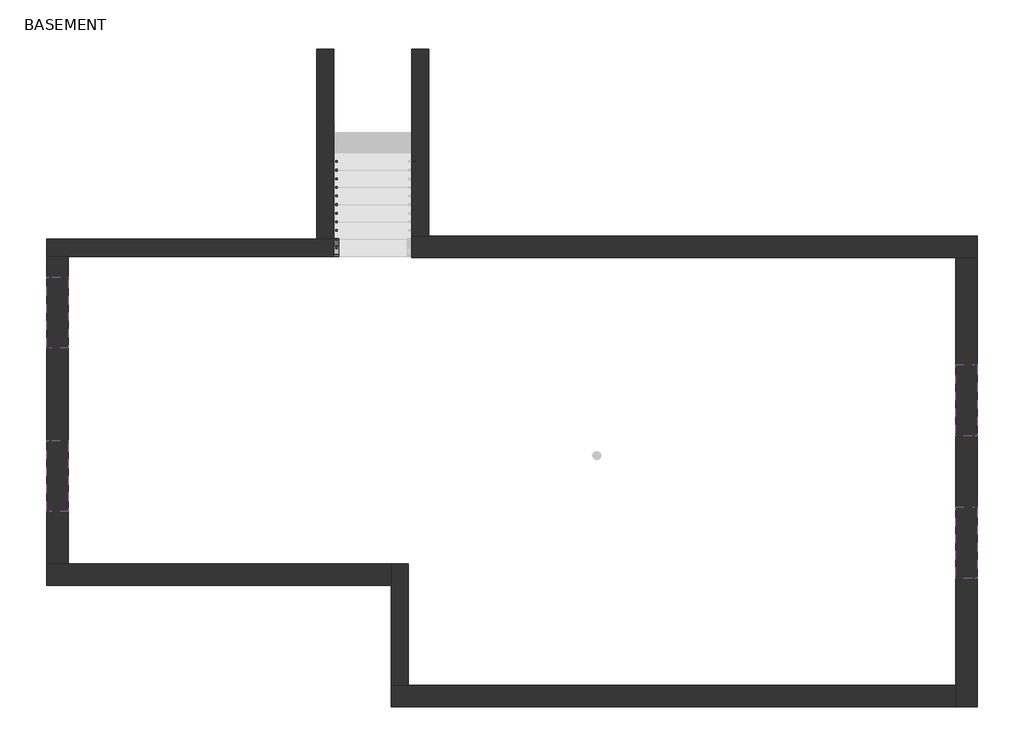
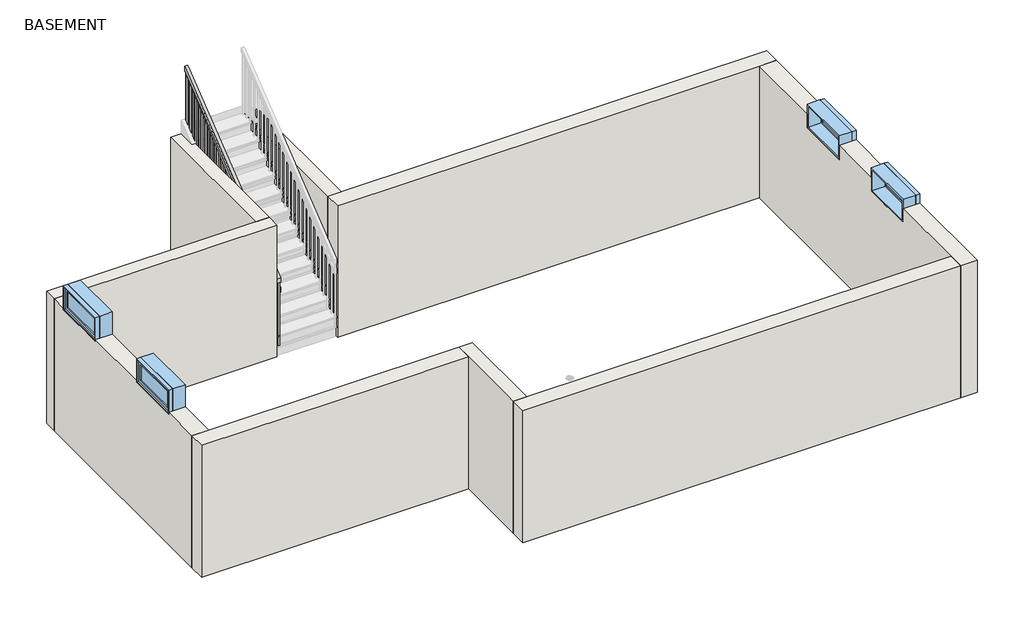
# One storey, part 1 of 2: 9 walls, 4 windows, 2 railings.
"""IFC4 building model written with IfcOpenShell, lengths in millimetres."""

import ifcopenshell
import ifcopenshell.guid

model = None  # the IFC model being written
_history = None  # IfcOwnerHistory: only IFC2X3 demands one
_inside = {}  # id of a spatial element -> (the spatial element, [elements in it])
_under = {}  # id of a project, library or spatial element -> (it, [spatial elements below it])
_declared = {}  # id of a project -> (the project, [libraries it declares])
_typed = {}  # id of a type object -> (the type object, [elements of that type])
_made_of = {}  # id of a material, layer set ... -> (it, [elements and type objects made of it])


def new_model(schema):
    """Start an empty IFC model of exactly this schema.

    Asked for "IFC4X3", IfcOpenShell would pick the latest addendum, in which some entities
    have other attributes; the version numbers below select the first issue.
    IFC2X3 requires an IfcOwnerHistory on every rooted entity: one is made here for all.
    """
    global model, _history
    if schema == "IFC4X3":
        model = ifcopenshell.file(schema_version=(4, 3, 0, 0))
    else:
        model = ifcopenshell.file(schema=schema)
    _inside.clear()
    _under.clear()
    _declared.clear()
    _typed.clear()
    _made_of.clear()
    _history = None
    if model.schema == "IFC2X3":
        org = make("IfcOrganization", Name="unknown")
        user = make(
            "IfcPersonAndOrganization",
            ThePerson=make("IfcPerson", FamilyName="unknown"),
            TheOrganization=org,
        )
        app = make(
            "IfcApplication",
            ApplicationDeveloper=org,
            Version="unknown",
            ApplicationFullName="unknown",
            ApplicationIdentifier="unknown",
        )
        _history = make(
            "IfcOwnerHistory",
            OwningUser=user,
            OwningApplication=app,
            ChangeAction="ADDED",
            CreationDate=0,
        )
    return model


def make(cls, **values):
    """One entity of the class cls with the attributes given. An attribute that is None is left unset."""
    return model.create_entity(
        cls, **{name: value for name, value in values.items() if value is not None}
    )


def rooted(cls, **values):
    """An entity with a GlobalId (a new one), such as an element, a storey or a relation."""
    return make(cls, GlobalId=ifcopenshell.guid.new(), OwnerHistory=_history, **values)


def si_unit(unit_type, name, prefix=None):
    """IfcSIUnit, for example si_unit("LENGTHUNIT", "METRE", prefix="MILLI")."""
    return make("IfcSIUnit", UnitType=unit_type, Prefix=prefix, Name=name)


def assignment(units):
    """IfcUnitAssignment: the units of a project."""
    return None if units is None else make("IfcUnitAssignment", Units=units)


def point(xyz):
    """IfcCartesianPoint."""
    return None if xyz is None else make("IfcCartesianPoint", Coordinates=xyz)


def direction(xyz):
    """IfcDirection."""
    return None if xyz is None else make("IfcDirection", DirectionRatios=xyz)


def frame(location, z_axis=None, x_axis=None):
    """IfcAxis2Placement3D, a coordinate frame: its origin and axes. An axis left out is left unset."""
    return make(
        "IfcAxis2Placement3D",
        Location=point(location),
        Axis=direction(z_axis),
        RefDirection=direction(x_axis),
    )


def origin():
    """The frame at (0, 0, 0) with its axes left unset."""
    return frame((0.0, 0.0, 0.0))


def place(relative_to, where):
    """IfcLocalPlacement: puts the frame where relative to a parent placement (None: the world)."""
    return make(
        "IfcLocalPlacement", PlacementRelTo=relative_to, RelativePlacement=where
    )


def context(
    kind, dimensions, precision=None, world=None, true_north=None, identifier=None
):
    """IfcGeometricRepresentationContext, for example the 3D "Model" context."""
    return make(
        "IfcGeometricRepresentationContext",
        ContextIdentifier=identifier,
        ContextType=kind,
        CoordinateSpaceDimension=dimensions,
        Precision=precision,
        WorldCoordinateSystem=world,
        TrueNorth=true_north,
    )


def project(units=None, contexts=None):
    """IfcProject with its units and contexts."""
    return rooted(
        "IfcProject",
        Name="project",
        RepresentationContexts=contexts,
        UnitsInContext=assignment(units),
    )


def spatial(cls, under=None, at=None, **own):
    """A site, building, storey or space (cls), placed at a placement, below another one or the project."""
    s = rooted(cls, ObjectPlacement=at, **own)
    if under is not None:
        _under.setdefault(under.id(), (under, []))[1].append(s)
    return s


def polyline(points):
    """IfcPolyline through the points."""
    return make("IfcPolyline", Points=[point(p) for p in points])


def outline(outer, holes=None, kind="AREA"):
    """IfcArbitraryClosedProfileDef: a profile drawn as a closed curve; with holes, ...WithVoids."""
    if holes is None:
        return make("IfcArbitraryClosedProfileDef", ProfileType=kind, OuterCurve=outer)
    return make(
        "IfcArbitraryProfileDefWithVoids",
        ProfileType=kind,
        OuterCurve=outer,
        InnerCurves=holes,
    )


def extrude(swept, where, along, depth):
    """IfcExtrudedAreaSolid: the profile swept, set in the frame where, extruded along a direction by depth."""
    return make(
        "IfcExtrudedAreaSolid",
        SweptArea=swept,
        Position=where,
        ExtrudedDirection=direction(along),
        Depth=depth,
    )


def faces_of(points, faces, orient=None, outer=None):
    """IfcFace entities. A face is a list of loops; a loop is a list of indices into points, from 0.

    orient and outer hold one flag for each loop. By default every Orientation is true, the
    first loop of a face is its IfcFaceOuterBound and the others are IfcFaceBound.
    """
    made = []
    for i, loops in enumerate(faces):
        bounds = []
        for j, loop in enumerate(loops):
            is_outer = j == 0 if outer is None else outer[i][j]
            bounds.append(
                make(
                    "IfcFaceOuterBound" if is_outer else "IfcFaceBound",
                    Bound=make("IfcPolyLoop", Polygon=[points[k] for k in loop]),
                    Orientation=True if orient is None else orient[i][j],
                )
            )
        made.append(make("IfcFace", Bounds=bounds))
    return made


def faceted_brep(points, faces, orient=None, outer=None, voids=None):
    """IfcFacetedBrep: a solid bounded by flat faces; with voids (closed shells), ...WithVoids."""
    shared = [point(p) for p in points]
    hull = make("IfcClosedShell", CfsFaces=faces_of(shared, faces, orient, outer))
    if voids is None:
        return make("IfcFacetedBrep", Outer=hull)
    return make(
        "IfcFacetedBrepWithVoids",
        Outer=hull,
        Voids=[
            make(cls, CfsFaces=faces_of(shared, fs, o, b)) for cls, fs, o, b in voids
        ],
    )


def shape(context_of_items, identifier, shape_type, items):
    """IfcShapeRepresentation: the items that make up one representation, for example the "Body"."""
    return make(
        "IfcShapeRepresentation",
        ContextOfItems=context_of_items,
        RepresentationIdentifier=identifier,
        RepresentationType=shape_type,
        Items=items,
    )


def source(mapping_origin, context_of_items, identifier, shape_type, items):
    """IfcRepresentationMap: a shape defined once, which mapped items show again and again."""
    return make(
        "IfcRepresentationMap",
        MappingOrigin=mapping_origin,
        MappedRepresentation=shape(context_of_items, identifier, shape_type, items),
    )


def transform(
    local_origin,
    x_axis=None,
    y_axis=None,
    z_axis=None,
    scale=None,
    scale2=None,
    scale3=None,
    uniform=True,
):
    """IfcCartesianTransformationOperator3D, or its non-uniform kind. x_axis, y_axis, z_axis: its Axis1, 2, 3."""
    if uniform:
        return make(
            "IfcCartesianTransformationOperator3D",
            Axis1=direction(x_axis),
            Axis2=direction(y_axis),
            LocalOrigin=point(local_origin),
            Scale=scale,
            Axis3=direction(z_axis),
        )
    return make(
        "IfcCartesianTransformationOperator3DnonUniform",
        Axis1=direction(x_axis),
        Axis2=direction(y_axis),
        LocalOrigin=point(local_origin),
        Scale=scale,
        Axis3=direction(z_axis),
        Scale2=scale2,
        Scale3=scale3,
    )


def mapped(mapping_source, mapping_target):
    """IfcMappedItem: shows the shape of a source again, moved by a transform."""
    return make(
        "IfcMappedItem", MappingSource=mapping_source, MappingTarget=mapping_target
    )


def made_of(thing, what):
    """Note that an element or type object is made of a material, layer set ...; save() writes the relation."""
    if what is not None:
        _made_of.setdefault(what.id(), (what, []))[1].append(thing)
    return thing


def element(
    cls,
    number,
    at=None,
    inside=None,
    cuts=None,
    type_object=None,
    material=None,
    context=None,
    identifier="Body",
    shape_type=None,
    held_by="IfcProductDefinitionShape",
    body=None,
    shapes=None,
    **own,
):
    """One element of the class cls, such as IfcWall. Its Tag is "e" and its number.

    at: its placement. inside: the storey or other place that contains it. cuts: it is an
    opening in that element (IfcRelVoidsElement). A single representation is given by context,
    identifier, shape_type and body (its items); several are given by shapes. held_by: the class
    of the entity that holds the representations. save() writes the other relations.
    """
    e = rooted(cls, Tag="e%d" % number, ObjectPlacement=at, **own)
    if body is not None:
        shapes = [shape(context, identifier, shape_type, body)]
    if shapes is not None:
        e.Representation = make(held_by, Representations=shapes)
    if inside is not None:
        _inside.setdefault(inside.id(), (inside, []))[1].append(e)
    if cuts is not None:
        rooted(
            "IfcRelVoidsElement", RelatingBuildingElement=cuts, RelatedOpeningElement=e
        )
    if type_object is not None:
        _typed.setdefault(type_object.id(), (type_object, []))[1].append(e)
    return made_of(e, material)


def aggregate(whole, parts):
    """IfcRelAggregates: a whole, such as a stair, and the parts it consists of."""
    return rooted("IfcRelAggregates", RelatingObject=whole, RelatedObjects=parts)


def save(model, path):
    """Write the relations noted so far, then the file.

    IfcRelAggregates (storeys below a building ...), IfcRelContainedInSpatialStructure (elements
    in a storey), IfcRelDefinesByType, IfcRelAssociatesMaterial and IfcRelDeclares: one each for
    every whole, place, type object, material and project.
    """
    for whole, parts in _under.values():
        aggregate(whole, parts)
    for where, things in _inside.values():
        rooted(
            "IfcRelContainedInSpatialStructure",
            RelatedElements=things,
            RelatingStructure=where,
        )
    for kind, things in _typed.values():
        rooted("IfcRelDefinesByType", RelatedObjects=things, RelatingType=kind)
    for what, things in _made_of.values():
        rooted("IfcRelAssociatesMaterial", RelatedObjects=things, RelatingMaterial=what)
    for by, libraries in _declared.values():
        rooted("IfcRelDeclares", RelatingContext=by, RelatedDefinitions=libraries)
    model.write(path)


def window_bf5cd34b(model_context):
    return source(origin(), model_context, "Body", "SweptSolid", [
        extrude(outline(polyline([(317.5, 79.375), (-393.7, 79.375), (-393.7, 92.075), (317.5, 92.075), (317.5, 79.375)])), frame((0.0, 0.0, 977.9), z_axis=(0.0, 0.0, 1.0), x_axis=(1.0, 0.0, 0.0)), (0.0, 0.0, 1.0), 254.0),
        extrude(outline(polyline([(1276.35, -438.15), (933.45, -438.15), (933.45, 361.95), (1276.35, 361.95), (1276.35, -438.15)]), holes=[polyline([(1231.9, -393.7), (1231.9, 317.5), (977.9, 317.5), (977.9, -393.7), (1231.9, -393.7)])]), frame((0.0, 63.5, 0.0), z_axis=(0.0, 1.0, 0.0), x_axis=(0.0, 0.0, 1.0)), (0.0, 0.0, 1.0), 44.45),
        extrude(outline(polyline([(1295.4, -457.2), (914.4, -457.2), (914.4, 381.0), (1295.4, 381.0), (1295.4, -457.2)]), holes=[polyline([(1263.65, -425.45), (1263.65, 349.25), (946.15, 349.25), (946.15, -425.45), (1263.65, -425.45)])]), frame((0.0, -127.0, 0.0), z_axis=(0.0, 1.0, 0.0), x_axis=(0.0, 0.0, 1.0)), (0.0, 0.0, 1.0), 190.5),
        extrude(outline(polyline([(1295.4, 381.0), (1295.4, -457.2), (914.4, -457.2), (914.4, 381.0), (1295.4, 381.0)]), holes=[polyline([(1276.35, 361.95), (933.45, 361.95), (933.45, -438.15), (1276.35, -438.15), (1276.35, 361.95)])]), frame((0.0, 63.5, 0.0), z_axis=(0.0, 1.0, 0.0), x_axis=(0.0, 0.0, 1.0)), (0.0, 0.0, 1.0), 63.5),
    ])


model = new_model("IFC4")

# Units and contexts
model_context = context("Model", 3, world=origin())
ifc_project = project(units=[si_unit("LENGTHUNIT", "METRE", prefix="MILLI")], contexts=[model_context])

# Site, building, storey
site = spatial("IfcSite", under=ifc_project)
building = spatial("IfcBuilding", under=site)
storey = spatial("IfcBuildingStorey", under=building, Name="BASEMENT", Elevation=-2266.95)

# Railings
placement = place(None, origin())
element("IfcRailing", 1, ObjectType="Handrail - Rectangular", at=placement, inside=storey, context=model_context, shape_type="SweptSolid", body=[
    extrude(outline(polyline([(-12572.2570712, -1084.7503866), (-12572.2570712, -1019.9076923), (-10133.8570712, 914.4), (-10133.8570712, 849.5573057), (-12572.2570712, -1084.7503866)])), frame((-25042.4664763, 0.0, 0.0), z_axis=(1.0, 0.0, 0.0), x_axis=(0.0, 1.0, 0.0)), (0.0, 0.0, 1.0), 50.8),
    extrude(outline(polyline([(-10225.9320712, 776.5170413), (-10225.9320712, -161.1923077), (-10244.9820712, -161.1923077), (-10244.9820712, 761.4052624), (-10225.9320712, 776.5170413)])), frame((-25026.5914763, 0.0, 0.0), z_axis=(1.0, 0.0, 0.0), x_axis=(0.0, 1.0, 0.0)), (0.0, 0.0, 1.0), 19.05),
    extrude(outline(polyline([(-10327.5320712, 695.9208874), (-10327.5320712, -161.1923077), (-10346.5820712, -161.1923077), (-10346.5820712, 680.8091086), (-10327.5320712, 695.9208874)])), frame((-25026.5914763, 0.0, 0.0), z_axis=(1.0, 0.0, 0.0), x_axis=(0.0, 1.0, 0.0)), (0.0, 0.0, 1.0), 19.05),
    extrude(outline(polyline([(-10429.1320712, 615.3247336), (-10429.1320712, -322.3846154), (-10448.1820712, -322.3846154), (-10448.1820712, 600.2129547), (-10429.1320712, 615.3247336)])), frame((-25026.5914763, 0.0, 0.0), z_axis=(1.0, 0.0, 0.0), x_axis=(0.0, 1.0, 0.0)), (0.0, 0.0, 1.0), 19.05),
    extrude(outline(polyline([(-10530.7320712, 534.7285797), (-10530.7320712, -322.3846154), (-10549.7820712, -322.3846154), (-10549.7820712, 519.6168009), (-10530.7320712, 534.7285797)])), frame((-25026.5914763, 0.0, 0.0), z_axis=(1.0, 0.0, 0.0), x_axis=(0.0, 1.0, 0.0)), (0.0, 0.0, 1.0), 19.05),
    extrude(outline(polyline([(-10632.3320712, 454.1324259), (-10632.3320712, -483.5769231), (-10651.3820712, -483.5769231), (-10651.3820712, 439.020647), (-10632.3320712, 454.1324259)])), frame((-25026.5914763, 0.0, 0.0), z_axis=(1.0, 0.0, 0.0), x_axis=(0.0, 1.0, 0.0)), (0.0, 0.0, 1.0), 19.05),
    extrude(outline(polyline([(-10733.9320712, 373.536272), (-10733.9320712, -483.5769231), (-10752.9820712, -483.5769231), (-10752.9820712, 358.4244932), (-10733.9320712, 373.536272)])), frame((-25026.5914763, 0.0, 0.0), z_axis=(1.0, 0.0, 0.0), x_axis=(0.0, 1.0, 0.0)), (0.0, 0.0, 1.0), 19.05),
    extrude(outline(polyline([(-10835.5320712, 292.9401182), (-10835.5320712, -644.7692308), (-10854.5820712, -644.7692308), (-10854.5820712, 277.8283394), (-10835.5320712, 292.9401182)])), frame((-25026.5914763, 0.0, 0.0), z_axis=(1.0, 0.0, 0.0), x_axis=(0.0, 1.0, 0.0)), (0.0, 0.0, 1.0), 19.05),
    extrude(outline(polyline([(-10937.1320712, 212.3439644), (-10937.1320712, -644.7692308), (-10956.1820712, -644.7692308), (-10956.1820712, 197.2321855), (-10937.1320712, 212.3439644)])), frame((-25026.5914763, 0.0, 0.0), z_axis=(1.0, 0.0, 0.0), x_axis=(0.0, 1.0, 0.0)), (0.0, 0.0, 1.0), 19.05),
    extrude(outline(polyline([(-11038.7320712, 131.7478105), (-11038.7320712, -805.9615385), (-11057.7820712, -805.9615385), (-11057.7820712, 116.6360317), (-11038.7320712, 131.7478105)])), frame((-25026.5914763, 0.0, 0.0), z_axis=(1.0, 0.0, 0.0), x_axis=(0.0, 1.0, 0.0)), (0.0, 0.0, 1.0), 19.05),
    extrude(outline(polyline([(-11140.3320712, 51.1516567), (-11140.3320712, -805.9615385), (-11159.3820712, -805.9615385), (-11159.3820712, 36.0398778), (-11140.3320712, 51.1516567)])), frame((-25026.5914763, 0.0, 0.0), z_axis=(1.0, 0.0, 0.0), x_axis=(0.0, 1.0, 0.0)), (0.0, 0.0, 1.0), 19.05),
    extrude(outline(polyline([(-11241.9320712, -29.4444972), (-11241.9320712, -967.1538462), (-11260.9820712, -967.1538462), (-11260.9820712, -44.556276), (-11241.9320712, -29.4444972)])), frame((-25026.5914763, 0.0, 0.0), z_axis=(1.0, 0.0, 0.0), x_axis=(0.0, 1.0, 0.0)), (0.0, 0.0, 1.0), 19.05),
    extrude(outline(polyline([(-11343.5320712, -110.040651), (-11343.5320712, -967.1538462), (-11362.5820712, -967.1538462), (-11362.5820712, -125.1524299), (-11343.5320712, -110.040651)])), frame((-25026.5914763, 0.0, 0.0), z_axis=(1.0, 0.0, 0.0), x_axis=(0.0, 1.0, 0.0)), (0.0, 0.0, 1.0), 19.05),
    extrude(outline(polyline([(-11445.1320712, -190.6368049), (-11445.1320712, -1128.3461538), (-11464.1820712, -1128.3461538), (-11464.1820712, -205.7485837), (-11445.1320712, -190.6368049)])), frame((-25026.5914763, 0.0, 0.0), z_axis=(1.0, 0.0, 0.0), x_axis=(0.0, 1.0, 0.0)), (0.0, 0.0, 1.0), 19.05),
    extrude(outline(polyline([(-11546.7320712, -271.2329587), (-11546.7320712, -1128.3461538), (-11565.7820712, -1128.3461538), (-11565.7820712, -286.3447376), (-11546.7320712, -271.2329587)])), frame((-25026.5914763, 0.0, 0.0), z_axis=(1.0, 0.0, 0.0), x_axis=(0.0, 1.0, 0.0)), (0.0, 0.0, 1.0), 19.05),
    extrude(outline(polyline([(-11648.3320712, -351.8291126), (-11648.3320712, -1289.5384615), (-11667.3820712, -1289.5384615), (-11667.3820712, -366.9408914), (-11648.3320712, -351.8291126)])), frame((-25026.5914763, 0.0, 0.0), z_axis=(1.0, 0.0, 0.0), x_axis=(0.0, 1.0, 0.0)), (0.0, 0.0, 1.0), 19.05),
    extrude(outline(polyline([(-11749.9320712, -432.4252664), (-11749.9320712, -1289.5384615), (-11768.9820712, -1289.5384615), (-11768.9820712, -447.5370453), (-11749.9320712, -432.4252664)])), frame((-25026.5914763, 0.0, 0.0), z_axis=(1.0, 0.0, 0.0), x_axis=(0.0, 1.0, 0.0)), (0.0, 0.0, 1.0), 19.05),
    extrude(outline(polyline([(-11851.5320712, -513.0214203), (-11851.5320712, -1450.7307692), (-11870.5820712, -1450.7307692), (-11870.5820712, -528.1331991), (-11851.5320712, -513.0214203)])), frame((-25026.5914763, 0.0, 0.0), z_axis=(1.0, 0.0, 0.0), x_axis=(0.0, 1.0, 0.0)), (0.0, 0.0, 1.0), 19.05),
    extrude(outline(polyline([(-11953.1320712, -593.6175741), (-11953.1320712, -1450.7307692), (-11972.1820712, -1450.7307692), (-11972.1820712, -608.729353), (-11953.1320712, -593.6175741)])), frame((-25026.5914763, 0.0, 0.0), z_axis=(1.0, 0.0, 0.0), x_axis=(0.0, 1.0, 0.0)), (0.0, 0.0, 1.0), 19.05),
    extrude(outline(polyline([(-12054.7320712, -674.213728), (-12054.7320712, -1611.9230769), (-12073.7820712, -1611.9230769), (-12073.7820712, -689.3255068), (-12054.7320712, -674.213728)])), frame((-25026.5914763, 0.0, 0.0), z_axis=(1.0, 0.0, 0.0), x_axis=(0.0, 1.0, 0.0)), (0.0, 0.0, 1.0), 19.05),
    extrude(outline(polyline([(-12156.3320712, -754.8098818), (-12156.3320712, -1611.9230769), (-12175.3820712, -1611.9230769), (-12175.3820712, -769.9216606), (-12156.3320712, -754.8098818)])), frame((-25026.5914763, 0.0, 0.0), z_axis=(1.0, 0.0, 0.0), x_axis=(0.0, 1.0, 0.0)), (0.0, 0.0, 1.0), 19.05),
    extrude(outline(polyline([(-12257.9320712, -835.4060356), (-12257.9320712, -1773.1153846), (-12276.9820712, -1773.1153846), (-12276.9820712, -850.5178145), (-12257.9320712, -835.4060356)])), frame((-25026.5914763, 0.0, 0.0), z_axis=(1.0, 0.0, 0.0), x_axis=(0.0, 1.0, 0.0)), (0.0, 0.0, 1.0), 19.05),
    extrude(outline(polyline([(-12359.5320712, -916.0021895), (-12359.5320712, -1773.1153846), (-12378.5820712, -1773.1153846), (-12378.5820712, -931.1139683), (-12359.5320712, -916.0021895)])), frame((-25026.5914763, 0.0, 0.0), z_axis=(1.0, 0.0, 0.0), x_axis=(0.0, 1.0, 0.0)), (0.0, 0.0, 1.0), 19.05),
    extrude(outline(polyline([(-12461.1320712, -996.5983433), (-12461.1320712, -1934.3076923), (-12480.1820712, -1934.3076923), (-12480.1820712, -1011.7101222), (-12461.1320712, -996.5983433)])), frame((-25026.5914763, 0.0, 0.0), z_axis=(1.0, 0.0, 0.0), x_axis=(0.0, 1.0, 0.0)), (0.0, 0.0, 1.0), 19.05),
    extrude(outline(polyline([(-10133.8570712, 849.5573057), (-10133.8570712, -161.1923077), (-10152.9070712, -161.1923077), (-10152.9070712, 834.4455269), (-10133.8570712, 849.5573057)])), frame((-25026.5914763, 0.0, 0.0), z_axis=(1.0, 0.0, 0.0), x_axis=(0.0, 1.0, 0.0)), (0.0, 0.0, 1.0), 19.05),
    extrude(outline(polyline([(-12553.2070712, -1069.6386078), (-12553.2070712, -1934.3076923), (-12572.2570712, -1934.3076923), (-12572.2570712, -1084.7503866), (-12553.2070712, -1069.6386078)])), frame((-25026.5914763, 0.0, 0.0), z_axis=(1.0, 0.0, 0.0), x_axis=(0.0, 1.0, 0.0)), (0.0, 0.0, 1.0), 19.05),
])
element("IfcRailing", 2, ObjectType="Handrail - Rectangular", at=placement, inside=storey, context=model_context, shape_type="SweptSolid", body=[
    extrude(outline(polyline([(-12572.2570712, -1245.110853), (-12572.2570712, -1178.1692308), (-10133.8570712, 914.4), (-10133.8570712, 847.4583777), (-12572.2570712, -1245.110853)])), frame((-25042.4664763, 0.0, 0.0), z_axis=(1.0, 0.0, 0.0), x_axis=(0.0, 1.0, 0.0)), (0.0, 0.0, 1.0), 50.8),
    extrude(outline(polyline([(-10225.9320712, 768.4420917), (-10225.9320712, -174.3807692), (-10244.9820712, -174.3807692), (-10244.9820712, 752.0938946), (-10225.9320712, 768.4420917)])), frame((-25026.5914763, 0.0, 0.0), z_axis=(1.0, 0.0, 0.0), x_axis=(0.0, 1.0, 0.0)), (0.0, 0.0, 1.0), 19.05),
    extrude(outline(polyline([(-10327.5320712, 681.2517071), (-10327.5320712, -174.3807692), (-10346.5820712, -174.3807692), (-10346.5820712, 664.9035099), (-10327.5320712, 681.2517071)])), frame((-25026.5914763, 0.0, 0.0), z_axis=(1.0, 0.0, 0.0), x_axis=(0.0, 1.0, 0.0)), (0.0, 0.0, 1.0), 19.05),
    extrude(outline(polyline([(-10429.1320712, 594.0613224), (-10429.1320712, -348.7615385), (-10448.1820712, -348.7615385), (-10448.1820712, 577.7131253), (-10429.1320712, 594.0613224)])), frame((-25026.5914763, 0.0, 0.0), z_axis=(1.0, 0.0, 0.0), x_axis=(0.0, 1.0, 0.0)), (0.0, 0.0, 1.0), 19.05),
    extrude(outline(polyline([(-10530.7320712, 506.8709378), (-10530.7320712, -348.7615385), (-10549.7820712, -348.7615385), (-10549.7820712, 490.5227407), (-10530.7320712, 506.8709378)])), frame((-25026.5914763, 0.0, 0.0), z_axis=(1.0, 0.0, 0.0), x_axis=(0.0, 1.0, 0.0)), (0.0, 0.0, 1.0), 19.05),
    extrude(outline(polyline([(-10632.3320712, 419.6805532), (-10632.3320712, -523.1423077), (-10651.3820712, -523.1423077), (-10651.3820712, 403.3323561), (-10632.3320712, 419.6805532)])), frame((-25026.5914763, 0.0, 0.0), z_axis=(1.0, 0.0, 0.0), x_axis=(0.0, 1.0, 0.0)), (0.0, 0.0, 1.0), 19.05),
    extrude(outline(polyline([(-10733.9320712, 332.4901686), (-10733.9320712, -523.1423077), (-10752.9820712, -523.1423077), (-10752.9820712, 316.1419715), (-10733.9320712, 332.4901686)])), frame((-25026.5914763, 0.0, 0.0), z_axis=(1.0, 0.0, 0.0), x_axis=(0.0, 1.0, 0.0)), (0.0, 0.0, 1.0), 19.05),
    extrude(outline(polyline([(-10835.5320712, 245.299784), (-10835.5320712, -697.5230769), (-10854.5820712, -697.5230769), (-10854.5820712, 228.9515869), (-10835.5320712, 245.299784)])), frame((-25026.5914763, 0.0, 0.0), z_axis=(1.0, 0.0, 0.0), x_axis=(0.0, 1.0, 0.0)), (0.0, 0.0, 1.0), 19.05),
    extrude(outline(polyline([(-10937.1320712, 158.1093994), (-10937.1320712, -697.5230769), (-10956.1820712, -697.5230769), (-10956.1820712, 141.7612022), (-10937.1320712, 158.1093994)])), frame((-25026.5914763, 0.0, 0.0), z_axis=(1.0, 0.0, 0.0), x_axis=(0.0, 1.0, 0.0)), (0.0, 0.0, 1.0), 19.05),
    extrude(outline(polyline([(-11038.7320712, 70.9190147), (-11038.7320712, -871.9038462), (-11057.7820712, -871.9038462), (-11057.7820712, 54.5708176), (-11038.7320712, 70.9190147)])), frame((-25026.5914763, 0.0, 0.0), z_axis=(1.0, 0.0, 0.0), x_axis=(0.0, 1.0, 0.0)), (0.0, 0.0, 1.0), 19.05),
    extrude(outline(polyline([(-11140.3320712, -16.2713699), (-11140.3320712, -871.9038462), (-11159.3820712, -871.9038462), (-11159.3820712, -32.619567), (-11140.3320712, -16.2713699)])), frame((-25026.5914763, 0.0, 0.0), z_axis=(1.0, 0.0, 0.0), x_axis=(0.0, 1.0, 0.0)), (0.0, 0.0, 1.0), 19.05),
    extrude(outline(polyline([(-11241.9320712, -103.4617545), (-11241.9320712, -1046.2846154), (-11260.9820712, -1046.2846154), (-11260.9820712, -119.8099516), (-11241.9320712, -103.4617545)])), frame((-25026.5914763, 0.0, 0.0), z_axis=(1.0, 0.0, 0.0), x_axis=(0.0, 1.0, 0.0)), (0.0, 0.0, 1.0), 19.05),
    extrude(outline(polyline([(-11343.5320712, -190.6521391), (-11343.5320712, -1046.2846154), (-11362.5820712, -1046.2846154), (-11362.5820712, -207.0003362), (-11343.5320712, -190.6521391)])), frame((-25026.5914763, 0.0, 0.0), z_axis=(1.0, 0.0, 0.0), x_axis=(0.0, 1.0, 0.0)), (0.0, 0.0, 1.0), 19.05),
    extrude(outline(polyline([(-11445.1320712, -277.8425237), (-11445.1320712, -1220.6653846), (-11464.1820712, -1220.6653846), (-11464.1820712, -294.1907208), (-11445.1320712, -277.8425237)])), frame((-25026.5914763, 0.0, 0.0), z_axis=(1.0, 0.0, 0.0), x_axis=(0.0, 1.0, 0.0)), (0.0, 0.0, 1.0), 19.05),
    extrude(outline(polyline([(-11546.7320712, -365.0329083), (-11546.7320712, -1220.6653846), (-11565.7820712, -1220.6653846), (-11565.7820712, -381.3811054), (-11546.7320712, -365.0329083)])), frame((-25026.5914763, 0.0, 0.0), z_axis=(1.0, 0.0, 0.0), x_axis=(0.0, 1.0, 0.0)), (0.0, 0.0, 1.0), 19.05),
    extrude(outline(polyline([(-11648.3320712, -452.2232929), (-11648.3320712, -1395.0461538), (-11667.3820712, -1395.0461538), (-11667.3820712, -468.5714901), (-11648.3320712, -452.2232929)])), frame((-25026.5914763, 0.0, 0.0), z_axis=(1.0, 0.0, 0.0), x_axis=(0.0, 1.0, 0.0)), (0.0, 0.0, 1.0), 19.05),
    extrude(outline(polyline([(-11749.9320712, -539.4136776), (-11749.9320712, -1395.0461538), (-11768.9820712, -1395.0461538), (-11768.9820712, -555.7618747), (-11749.9320712, -539.4136776)])), frame((-25026.5914763, 0.0, 0.0), z_axis=(1.0, 0.0, 0.0), x_axis=(0.0, 1.0, 0.0)), (0.0, 0.0, 1.0), 19.05),
    extrude(outline(polyline([(-11851.5320712, -626.6040622), (-11851.5320712, -1569.4269231), (-11870.5820712, -1569.4269231), (-11870.5820712, -642.9522593), (-11851.5320712, -626.6040622)])), frame((-25026.5914763, 0.0, 0.0), z_axis=(1.0, 0.0, 0.0), x_axis=(0.0, 1.0, 0.0)), (0.0, 0.0, 1.0), 19.05),
    extrude(outline(polyline([(-11953.1320712, -713.7944468), (-11953.1320712, -1569.4269231), (-11972.1820712, -1569.4269231), (-11972.1820712, -730.1426439), (-11953.1320712, -713.7944468)])), frame((-25026.5914763, 0.0, 0.0), z_axis=(1.0, 0.0, 0.0), x_axis=(0.0, 1.0, 0.0)), (0.0, 0.0, 1.0), 19.05),
    extrude(outline(polyline([(-12054.7320712, -800.9848314), (-12054.7320712, -1743.8076923), (-12073.7820712, -1743.8076923), (-12073.7820712, -817.3330285), (-12054.7320712, -800.9848314)])), frame((-25026.5914763, 0.0, 0.0), z_axis=(1.0, 0.0, 0.0), x_axis=(0.0, 1.0, 0.0)), (0.0, 0.0, 1.0), 19.05),
    extrude(outline(polyline([(-12156.3320712, -888.175216), (-12156.3320712, -1743.8076923), (-12175.3820712, -1743.8076923), (-12175.3820712, -904.5234131), (-12156.3320712, -888.175216)])), frame((-25026.5914763, 0.0, 0.0), z_axis=(1.0, 0.0, 0.0), x_axis=(0.0, 1.0, 0.0)), (0.0, 0.0, 1.0), 19.05),
    extrude(outline(polyline([(-12257.9320712, -975.3656006), (-12257.9320712, -1918.1884615), (-12276.9820712, -1918.1884615), (-12276.9820712, -991.7137978), (-12257.9320712, -975.3656006)])), frame((-25026.5914763, 0.0, 0.0), z_axis=(1.0, 0.0, 0.0), x_axis=(0.0, 1.0, 0.0)), (0.0, 0.0, 1.0), 19.05),
    extrude(outline(polyline([(-12359.5320712, -1062.5559853), (-12359.5320712, -1918.1884615), (-12378.5820712, -1918.1884615), (-12378.5820712, -1078.9041824), (-12359.5320712, -1062.5559853)])), frame((-25026.5914763, 0.0, 0.0), z_axis=(1.0, 0.0, 0.0), x_axis=(0.0, 1.0, 0.0)), (0.0, 0.0, 1.0), 19.05),
    extrude(outline(polyline([(-12461.1320712, -1149.7463699), (-12461.1320712, -2092.5692308), (-12480.1820712, -2092.5692308), (-12480.1820712, -1166.094567), (-12461.1320712, -1149.7463699)])), frame((-25026.5914763, 0.0, 0.0), z_axis=(1.0, 0.0, 0.0), x_axis=(0.0, 1.0, 0.0)), (0.0, 0.0, 1.0), 19.05),
    extrude(outline(polyline([(-10133.8570712, 847.4583777), (-10133.8570712, -174.3807692), (-10152.9070712, -174.3807692), (-10152.9070712, 831.1101806), (-10133.8570712, 847.4583777)])), frame((-25026.5914763, 0.0, 0.0), z_axis=(1.0, 0.0, 0.0), x_axis=(0.0, 1.0, 0.0)), (0.0, 0.0, 1.0), 19.05),
    extrude(outline(polyline([(-12553.2070712, -1228.7626559), (-12553.2070712, -2092.5692308), (-12572.2570712, -2092.5692308), (-12572.2570712, -1245.110853), (-12553.2070712, -1228.7626559)])), frame((-25026.5914763, 0.0, 0.0), z_axis=(1.0, 0.0, 0.0), x_axis=(0.0, 1.0, 0.0)), (0.0, 0.0, 1.0), 19.05),
])

# Walls
element("IfcWall", 3, ObjectType="Generic - 10\"", at=placement, inside=storey, context=model_context, shape_type="Brep", body=[
    faceted_brep([(-17733.6164763, -12584.9570712, -2266.95), (-17733.6164763, -17620.5070712, -2266.95), (-17733.6164763, -17874.5070712, -2266.95), (-17733.6164763, -17874.5070712, -152.4), (-17733.6164763, -17620.5070712, -152.4), (-17733.6164763, -16361.0904046, -152.4), (-17733.6164763, -16361.0904046, -381.0), (-17733.6164763, -15522.8904046, -381.0), (-17733.6164763, -15522.8904046, -152.4), (-17733.6164763, -14682.5737379, -152.4), (-17733.6164763, -14682.5737379, -381.0), (-17733.6164763, -13844.3737379, -381.0), (-17733.6164763, -13844.3737379, -152.4), (-17733.6164763, -12584.9570712, -152.4), (-17479.6164763, -17874.5070712, -2266.95), (-17479.6164763, -12584.9570712, -2266.95), (-17479.6164763, -12584.9570712, -152.4), (-17479.6164763, -13844.3737379, -152.4), (-17479.6164763, -13844.3737379, -381.0), (-17479.6164763, -14682.5737379, -381.0), (-17479.6164763, -14682.5737379, -152.4), (-17479.6164763, -15522.8904046, -152.4), (-17479.6164763, -15522.8904046, -381.0), (-17479.6164763, -16361.0904046, -381.0), (-17479.6164763, -16361.0904046, -152.4), (-17479.6164763, -17874.5070712, -152.4)], [[[0, 1, 2, 3, 4, 5, 6, 7, 8, 9, 10, 11, 12, 13]], [[14, 15, 16, 17, 18, 19, 20, 21, 22, 23, 24, 25]], [[2, 1, 0, 15, 14]], [[0, 13, 16, 15]], [[3, 2, 14, 25]], [[3, 25, 24, 5, 4]], [[8, 21, 20, 9]], [[16, 13, 12, 17]], [[23, 6, 5, 24]], [[6, 23, 22, 7]], [[7, 22, 21, 8]], [[19, 10, 9, 20]], [[10, 19, 18, 11]], [[11, 18, 17, 12]]]),
])
element("IfcWall", 4, ObjectType="Generic - 10\"", at=placement, inside=storey, context=model_context, shape_type="Brep", body=[
    faceted_brep([(-17733.6164763, -17620.5070712, -2266.95), (-24172.5164763, -17620.5070712, -2266.95), (-24375.7164763, -17620.5070712, -2266.95), (-24375.7164763, -17620.5070712, -152.4), (-24172.5164763, -17620.5070712, -152.4), (-17733.6164763, -17620.5070712, -152.4), (-17733.6164763, -17874.5070712, -2266.95), (-17733.6164763, -17874.5070712, -152.4), (-24375.7164763, -17874.5070712, -152.4), (-24375.7164763, -17874.5070712, -2266.95)], [[[0, 1, 2, 3, 4, 5]], [[6, 7, 8, 9]], [[2, 1, 0, 6, 9]], [[0, 5, 7, 6]], [[3, 2, 9, 8]], [[5, 4, 3, 8, 7]]]),
])
element("IfcWall", 5, ObjectType="Generic - 10\"", at=placement, inside=storey, context=model_context, shape_type="Brep", body=[
    faceted_brep([(-24375.7164763, -16191.7570712, -2266.95), (-28173.0164763, -16191.7570712, -2266.95), (-28427.0164763, -16191.7570712, -2266.95), (-28427.0164763, -16191.7570712, -152.4), (-28173.0164763, -16191.7570712, -152.4), (-24375.7164763, -16191.7570712, -152.4), (-24375.7164763, -16445.7570712, -2266.95), (-24375.7164763, -16445.7570712, -152.4), (-25734.6164763, -16445.7570712, -152.4), (-28427.0164763, -16445.7570712, -152.4), (-28427.0164763, -16445.7570712, -2266.95)], [[[0, 1, 2, 3, 4, 5]], [[6, 7, 8, 9, 10]], [[2, 1, 0, 6, 10]], [[0, 5, 7, 6]], [[3, 2, 10, 9]], [[5, 4, 3, 9, 8, 7]]]),
])
element("IfcWall", 6, ObjectType="Generic - 10\"", at=placement, inside=storey, context=model_context, shape_type="SweptSolid", body=[
    extrude(outline(polyline([(-12572.2570712, -2266.95), (-16191.7570712, -2266.95), (-16191.7570712, -152.4), (-15575.8070712, -152.4), (-15575.8070712, -177.7746), (-14737.6070712, -177.7746), (-14737.6070712, -152.4), (-13651.7570712, -152.4), (-13651.7570712, -177.7746), (-12813.5570712, -177.7746), (-12813.5570712, -152.4), (-12572.2570712, -152.4), (-12572.2570712, -2266.95)])), frame((-28427.0164763, 0.0, 0.0), z_axis=(1.0, 0.0, 0.0), x_axis=(0.0, 1.0, 0.0)), (0.0, 0.0, 1.0), 254.0),
])
element("IfcWall", 7, ObjectType="Generic - 10\"", at=placement, inside=storey, context=model_context, shape_type="Brep", body=[
    faceted_brep([(-24134.4164763, -12584.9570712, -2266.95), (-17733.6164763, -12584.9570712, -2266.95), (-17479.6164763, -12584.9570712, -2266.95), (-17479.6164763, -12584.9570712, -152.4), (-17733.6164763, -12584.9570712, -152.4), (-24134.4164763, -12584.9570712, -152.4), (-24134.4164763, -12330.9570712, -2266.95), (-24134.4164763, -12330.9570712, -152.4), (-23931.2164763, -12330.9570712, -152.4), (-17479.6164763, -12330.9570712, -152.4), (-17479.6164763, -12330.9570712, -2266.95), (-23931.2164763, -12330.9570712, -2266.95)], [[[0, 1, 2, 3, 4, 5]], [[6, 7, 8, 9, 10, 11]], [[2, 1, 0, 6, 11, 10]], [[3, 2, 10, 9]], [[0, 5, 7, 6]], [[5, 4, 3, 9, 8, 7]]]),
])
element("IfcWall", 8, ObjectType="Generic - 8\"", at=placement, inside=storey, context=model_context, shape_type="Brep", body=[
    faceted_brep([(-28427.0164763, -12572.2570712, -2266.95), (-28173.0164763, -12572.2570712, -2266.95), (-25048.8164763, -12572.2570712, -2266.95), (-25048.8164763, -12572.2570712, -152.4), (-28173.0164763, -12572.2570712, -152.4), (-28427.0164763, -12572.2570712, -152.4), (-28427.0164763, -12369.0570712, -2266.95), (-28427.0164763, -12369.0570712, -152.4), (-25252.0164763, -12369.0570712, -152.4), (-25048.8164763, -12369.0570712, -152.4), (-25048.8164763, -12369.0570712, -2266.95), (-25252.0164763, -12369.0570712, -2266.95)], [[[0, 1, 2, 3, 4, 5]], [[6, 7, 8, 9, 10, 11]], [[2, 1, 0, 6, 11, 10]], [[0, 5, 7, 6]], [[3, 2, 10, 9]], [[5, 4, 3, 9, 8, 7]]]),
])
element("IfcWall", 9, ObjectType="Generic - 8\"", at=placement, inside=storey, context=model_context, shape_type="Brep", body=[
    faceted_brep([(-24172.5164763, -17620.5070712, -2266.95), (-24172.5164763, -16191.7570712, -2266.95), (-24172.5164763, -16191.7570712, -152.4), (-24172.5164763, -17620.5070712, -152.4), (-24375.7164763, -17620.5070712, -2266.95), (-24375.7164763, -17620.5070712, -152.4), (-24375.7164763, -16445.7570712, -152.4), (-24375.7164763, -16191.7570712, -152.4), (-24375.7164763, -16191.7570712, -2266.95), (-24375.7164763, -16445.7570712, -2266.95)], [[[0, 1, 2, 3]], [[4, 5, 6, 7, 8, 9]], [[1, 0, 4, 9, 8]], [[0, 3, 5, 4]], [[2, 1, 8, 7]], [[3, 2, 7, 6, 5]]]),
])
element("IfcWall", 10, ObjectType="Generic - 8\"", at=placement, inside=storey, context=model_context, shape_type="SweptSolid", body=[
    extrude(outline(polyline([(-25048.8164763, -10133.8570712), (-25048.8164763, -12369.0570712), (-25252.0164763, -12369.0570712), (-25252.0164763, -10133.8570712), (-25048.8164763, -10133.8570712)])), frame((0.0, 0.0, -2266.95), z_axis=(0.0, 0.0, 1.0), x_axis=(1.0, 0.0, 0.0)), (0.0, 0.0, 1.0), 2114.55),
])
element("IfcWall", 11, ObjectType="Generic - 8\"", at=placement, inside=storey, context=model_context, shape_type="SweptSolid", body=[
    extrude(outline(polyline([(-24134.4164763, -12330.9570712), (-24134.4164763, -10133.8570712), (-23931.2164763, -10133.8570712), (-23931.2164763, -12330.9570712), (-24134.4164763, -12330.9570712)])), frame((0.0, 0.0, -2266.95), z_axis=(0.0, 0.0, 1.0), x_axis=(1.0, 0.0, 0.0)), (0.0, 0.0, 1.0), 2114.55),
])

# Windows
window_shape = window_bf5cd34b(model_context)
element("IfcWindow", 12, ObjectType="Fixed1 : 2'-9\" x 1'-3\"", at=placement, inside=storey, context=model_context, shape_type="MappedRepresentation", body=[
    mapped(window_shape, transform((-28300.0164763, -15118.6070712, -1092.1746), x_axis=(0.0, 1.0, 0.0), y_axis=(-1.0, 0.0, 0.0), z_axis=(0.0, 0.0, 1.0))),
])
element("IfcWindow", 13, ObjectType="Fixed1 : 2'-9\" x 1'-3\"", at=placement, inside=storey, context=model_context, shape_type="MappedRepresentation", body=[
    mapped(window_shape, transform((-28300.0164763, -13194.5570712, -1092.1746), x_axis=(0.0, 1.0, 0.0), y_axis=(-1.0, 0.0, 0.0), z_axis=(0.0, 0.0, 1.0))),
])
element("IfcWindow", 14, ObjectType="Fixed1 : 2'-9\" x 1'-3\"", at=placement, inside=storey, context=model_context, shape_type="MappedRepresentation", body=[
    mapped(window_shape, transform((-17606.6164763, -14301.5737379, -1295.4), x_axis=(0.0, -1.0, 0.0), y_axis=(1.0, 0.0, 0.0), z_axis=(0.0, 0.0, 1.0))),
])
element("IfcWindow", 15, ObjectType="Fixed1 : 2'-9\" x 1'-3\"", at=placement, inside=storey, context=model_context, shape_type="MappedRepresentation", body=[
    mapped(window_shape, transform((-17606.6164763, -15980.0904046, -1295.4), x_axis=(0.0, -1.0, 0.0), y_axis=(1.0, 0.0, 0.0), z_axis=(0.0, 0.0, 1.0))),
])

save(model, "model.ifc")

# Revit data of these elements
# Project information
#   Project Issue Date = "06/12/2018"
#   Project Status = "Project Status"
#   Client Name = "Owner"
#   Project Address = "5253 KING JAMES WAY, FITCHBURG, WI"
#   Project Name = "FORAGE KOMBUCHA"
#   Project Number = "Project Number"
# Grids (mm)
#   "B": line (-20559.366, -20036.147) -> (-20559.366, -11545.141)
#   "C": line (-23277.166, -20036.147) -> (-23277.166, -11545.141)
#   "D": line (-25994.966, -20036.147) -> (-25994.966, -11545.141)
# Type "Handrail - Rectangular"
#   Assembly Code = "C2010400"
#   built-in parameter 1008612 = 0.0416667 (stored number, unit not read)
#   built-in parameter 1008611 = 0.0416667 (stored number, unit not read)
#   built-in parameter 1008609 = 0.333333 (stored number, unit not read)
#   built-in parameter 1008604 = 0.166667 (stored number, unit not read)
#   built-in parameter 1008603 = 0.166667 (stored number, unit not read)
#   Railing Height = 3' - 0"
#   built-in parameter 1008630 = 2
#   built-in parameter 1008610 = 2
#   built-in parameter 1008618 = Baluster - Square : 3/4"
# Type "Generic - 10\""
#   Assembly Code = "B2010"
#   Layers, outside or top first: 0' - 10" no material (function 1)
# Type "Generic - 8\""
#   Assembly Code = "B2010"
#   Layers, outside or top first: 0' - 8" no material (function 1)
# Type "Fixed1 : 2'-9\" x 1'-3\""
#   Type Mark = "29"
#   Construction Type Id = "GSP4R"
#   Assembly Code = "B2020100"
#   Analytic Construction = "1/8 in Pilkington single glazing"
#   Visual Light Transmittance = 0.9
#   Solar Heat Gain Coefficient = 0.78
#   Heat Transfer Coefficient (U) = 3.6886 W/(m²·K)
#   Height = 1' - 3"
#   Default Sill Height = 3' - 0"
#   Width = 2' - 9"
#   Window Inset = 0' - 0 3/4"
#   Glass Pane Material = Glass
#   Sash Material = Sash
#   Wall Closure = (empty or 0)
# Elements 1, 2 (IfcRailing, "Handrail - Rectangular")
#   Phase Created = 1st Phase
# Elements 3, 4, 5, 6, 7 (IfcWall, "Generic - 10\"")
#   Top Offset = 0' - 0"
#   Base Offset = 0' - 0"
#   wall height = 6' - 11 1/4"
#   Phase Created = 1st Phase
#   Base Constraint = BASEMENT
#   Top Constraint = 1ST FLOOR
# Elements 8, 9, 10, 11 (IfcWall, "Generic - 8\"")
#   Top Offset = 0' - 0"
#   Base Offset = 0' - 0"
#   wall height = 6' - 11 1/4"
#   Phase Created = 1st Phase
#   Base Constraint = BASEMENT
#   Top Constraint = 1ST FLOOR
# Element 12 (IfcWindow, "Fixed1 : 2'-9\" x 1'-3\"")
#   Mark = "26"
#   Phase Created = 1st Phase
#   Materials on its faces: "Sash", "Glass"
# Element 13 (IfcWindow, "Fixed1 : 2'-9\" x 1'-3\"")
#   Mark = "27"
#   Phase Created = 1st Phase
#   Materials on its faces: "Sash", "Glass"
# Element 14 (IfcWindow, "Fixed1 : 2'-9\" x 1'-3\"")
#   Mark = "28"
#   Phase Created = 1st Phase
#   Materials on its faces: "Sash", "Glass"
# Element 15 (IfcWindow, "Fixed1 : 2'-9\" x 1'-3\"")
#   Mark = "29"
#   Phase Created = 1st Phase
#   Materials on its faces: "Sash", "Glass"
# Materials
#   "Glass": class "Glass", colour RGB 218 227 224, transparency 0.85, Description = "Soda Lime Glass", Cost = 0
#   "Sash": class "Wood", colour RGB 224 178 126, transparency 0, Cost = 0
